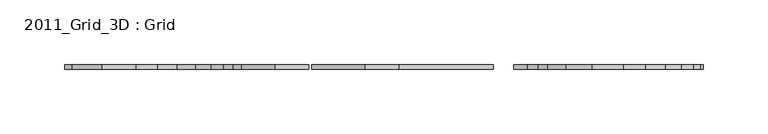
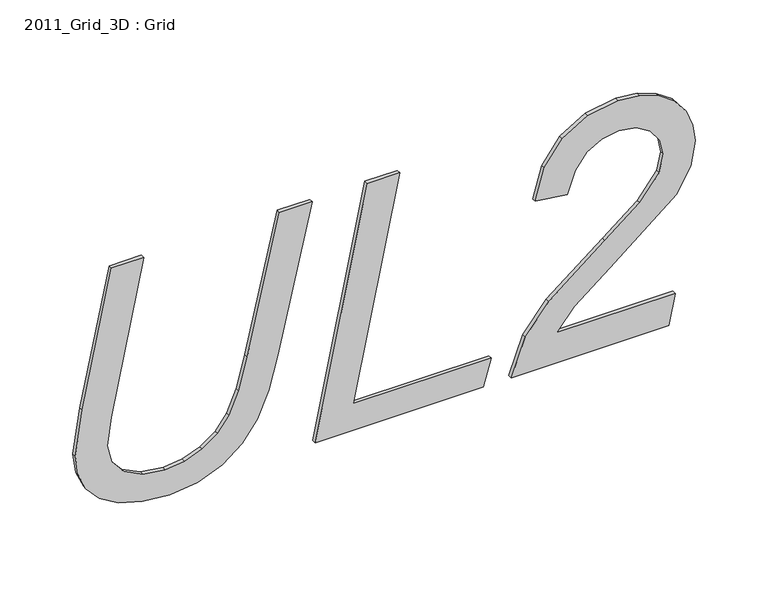
"""IFC4 building model written with IfcOpenShell, lengths in millimetres: proxy geometry, 2011_Grid_3D : Grid."""

from ifc_helpers import new_model, si_unit, frame, origin, place, context, project, spatial, polyline, outline, extrude, source, transform, mapped, element, save


def proxy_2011_grid_3d_grid_2471bd22(model_context):
    return source(origin(), model_context, "Body", "SweptSolid", [
        extrude(outline(polyline([(101.4447294, 47277.8299768), (-9.5457855, 47254.7296731), (-46.3278141, 47249.0785258), (-62.2836301, 47251.2224918), (-76.4424804, 47257.6543897), (-88.2714718, 47268.3866123), (-97.2377109, 47283.4315526), (-102.8888581, 47302.2191386), (-104.7725739, 47324.1792986), (-102.1081075, 47346.374923), (-94.1147085, 47365.6706165), (-81.7032524, 47381.5706646), (-65.784615, 47393.5793525), (-44.9584024, 47402.6757168), (-17.8242205, 47409.8387938), (101.4447294, 47437.0039577), (101.4447294, 47411.0780804), (-10.7355007, 47385.4992034), (-36.7791103, 47378.8070553), (-54.6310349, 47371.3217638), (-66.7202764, 47362.0271137), (-75.4758368, 47349.90689), (-80.7923767, 47335.8285933), (-82.5645566, 47320.6597244), (-80.0983761, 47302.5599424), (-72.6998347, 47287.8186274), (-61.2488258, 47278.0220662), (-46.6252429, 47274.7565458), (-23.5745107, 47277.8795482), (101.4447294, 47303.5575682), (101.4447294, 47277.8299768)])), frame((0.0, -3.175, 0.0), z_axis=(0.0, 1.0, 0.0), x_axis=(0.0, 0.0, 1.0)), (0.0, 0.0, 1.0), 3.175),
        extrude(outline(polyline([(-101.6, 47439.4329596), (-101.6, 47572.6810633), (-79.3919827, 47579.0262111), (-79.3919827, 47469.7211261), (101.4447294, 47506.4535832), (101.4447294, 47480.6764203), (-101.6, 47439.4329596)])), frame((0.0, -3.175, 0.0), z_axis=(0.0, 1.0, 0.0), x_axis=(0.0, 0.0, 1.0)), (0.0, 0.0, 1.0), 3.175),
        extrude(outline(polyline([(-101.6, 47594.8890806), (-101.6, 47719.9578921), (-76.2194088, 47724.9646103), (-76.2194088, 47631.0762516), (-59.4146815, 47644.9810481), (-36.6118066, 47673.1128557), (6.8127986, 47726.1543255), (26.1828494, 47737.1591912), (46.3212579, 47740.8274798), (60.1826794, 47739.0181213), (73.6103506, 47733.5900456), (85.3463954, 47724.5618422), (94.132938, 47711.9521002), (99.6167815, 47696.7150705), (101.4447294, 47679.8050038), (97.3302976, 47655.4220384), (84.9870023, 47635.4137549), (65.5054157, 47621.130976), (39.9761101, 47613.9245239), (36.6052504, 47639.3051151), (54.4881571, 47645.5325307), (66.6951309, 47654.8953415), (73.7218864, 47666.7367257), (76.0641382, 47680.3998614), (73.7528686, 47694.0134255), (66.8190596, 47705.3095236), (56.5763552, 47712.9125474), (44.3383992, 47715.4468886), (29.7643879, 47712.1751718), (9.6879437, 47696.7584455), (-12.2226448, 47669.2462813), (-47.7901724, 47624.5080322), (-71.1135477, 47605.8691605), (-101.6, 47594.8890806)])), frame((0.0, -3.175, 0.0), z_axis=(0.0, 1.0, 0.0), x_axis=(0.0, 0.0, 1.0)), (0.0, 0.0, 1.0), 3.175),
    ])


if __name__ == "__main__":
    model = new_model("IFC4")
    model_context = context("Model", 3, world=origin())
    ifc_project = project(units=[si_unit("LENGTHUNIT", "METRE", prefix="MILLI")], contexts=[model_context])
    site = spatial("IfcSite", under=ifc_project)
    building = spatial("IfcBuilding", under=site)
    placement = place(None, origin())
    proxy_2011_grid_3d_grid_shape = proxy_2011_grid_3d_grid_2471bd22(model_context)
    element("IfcBuildingElementProxy", 1, Name="2011_Grid_3D : Grid", ObjectType="2011_Grid_3D : Grid", at=placement, inside=building, context=model_context, shape_type="MappedRepresentation", body=[
        mapped(proxy_2011_grid_3d_grid_shape, transform((0.0, 0.0, 0.0), x_axis=(1.0, 0.0, 0.0), y_axis=(0.0, 1.0, 0.0), z_axis=(0.0, 0.0, 1.0))),
    ])
    save(model, "model.ifc")

# Revit data of these elements
# Type "2011_Grid_3D : Grid"
#   Workplane [instance default] = "LEVEL"
#   Grid [instance default] = "S"
#   t [instance default] = 12' - 6"
#   built-in parameter 1001306 [instance default] = 50 (stored number, unit not read)
#   d [instance default] = 2
#   Symbol At End 2 [instance default] = yes
#   Symbol At End 1 [instance default] = yes
#   Robust [instance default] = yes
#   No of grid markers [instance default] = 3
#   Grid Height Visible = yes
#   Height = 0
#   Assembly Code = ""
# Element 1 (IfcBuildingElementProxy, "2011_Grid_3D : Grid")
#   Workplane = "UL2"
#   Grid = "A"
#   t = 11' - 0.37148"
#   built-in parameter 1001306 = 154.433 (stored number, unit not read)
#   d = 7
#   Robust = no
#   No of grid markers = 8
#   Materials on its faces: "Letter"
# Materials
#   "Letter": class "Unassigned", colour RGB 178 187 30, transparency 0, Comments = "Rendering appearance not upgraded "
